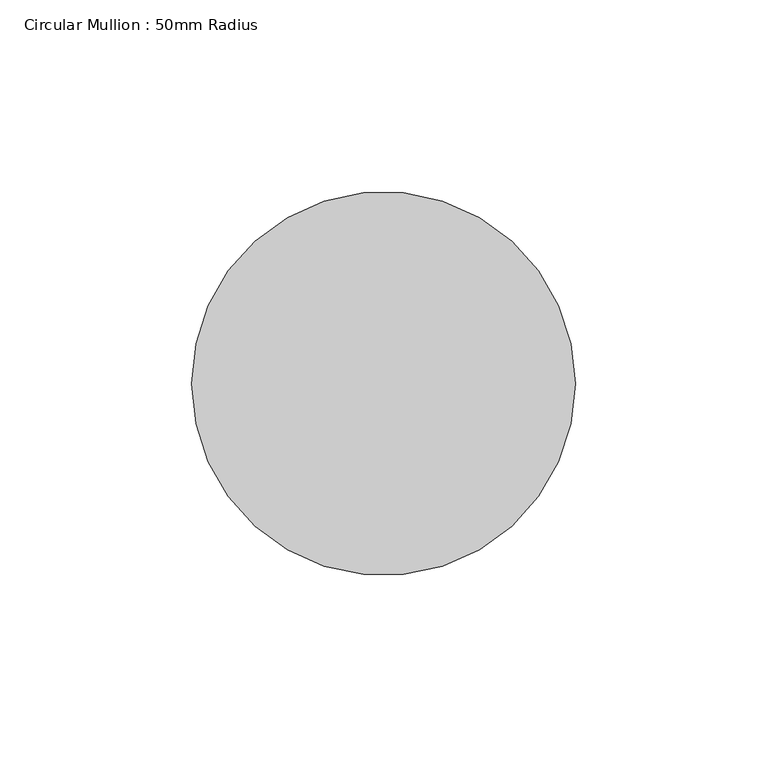
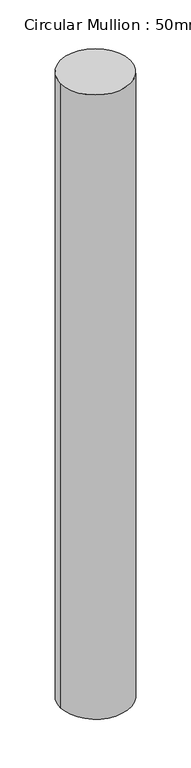
"""IFC4 building model written with IfcOpenShell, lengths in millimetres: member geometry, Circular Mullion : 50mm Radius."""

from ifc_helpers import new_model, si_unit, point, frame, origin, origin_2d, place, context, project, spatial, circle_curve, trimmed, segment, composite_curve, outline, extrude, source, transform, mapped, element, save


def circular_mullion_50mm_radius_4ee3f7eb(model_context):
    return source(origin(), model_context, "Body", "SweptSolid", [
        extrude(outline(composite_curve([segment(trimmed(circle_curve(origin_2d(), 50.0), [point((50.0, 0.0))], [point((-50.0, 0.0))], False, "CARTESIAN"), True, "CONTINUOUS"), segment(trimmed(circle_curve(origin_2d(), 50.0), [point((-50.0, 0.0))], [point((50.0, 0.0))], False, "CARTESIAN"), True, "CONTINUOUS")], self_intersect=False)), frame((0.0, 0.0, -945.3930729), z_axis=(0.0, 0.0, 1.0), x_axis=(1.0, 0.0, 0.0)), (0.0, 0.0, 1.0), 945.3930729),
    ])


if __name__ == "__main__":
    model = new_model("IFC4")
    model_context = context("Model", 3, world=origin())
    ifc_project = project(units=[si_unit("LENGTHUNIT", "METRE", prefix="MILLI")], contexts=[model_context])
    site = spatial("IfcSite", under=ifc_project)
    building = spatial("IfcBuilding", under=site)
    placement = place(None, origin())
    circular_mullion_50mm_radius_shape = circular_mullion_50mm_radius_4ee3f7eb(model_context)
    element("IfcMember", 1, ObjectType="Circular Mullion : 50mm Radius", at=placement, inside=building, context=model_context, shape_type="MappedRepresentation", body=[
        mapped(circular_mullion_50mm_radius_shape, transform((0.0, 0.0, 0.0), x_axis=(1.0, 0.0, 0.0), y_axis=(0.0, 1.0, 0.0), z_axis=(0.0, 0.0, 1.0))),
    ])
    save(model, "model.ifc")

# Revit data of these elements
# Type "Circular Mullion : 50mm Radius"
#   built-in parameter 1007350 = 0.164042 (stored number, unit not read)
# Element 1 (IfcMember, "Circular Mullion : 50mm Radius")
#   Materials on its faces: "Aluminium"
# Materials
#   "Aluminium": class "Metal", colour RGB 247 247 247, transparency 0, Description = "Aluminium 6061", Cost = 0
